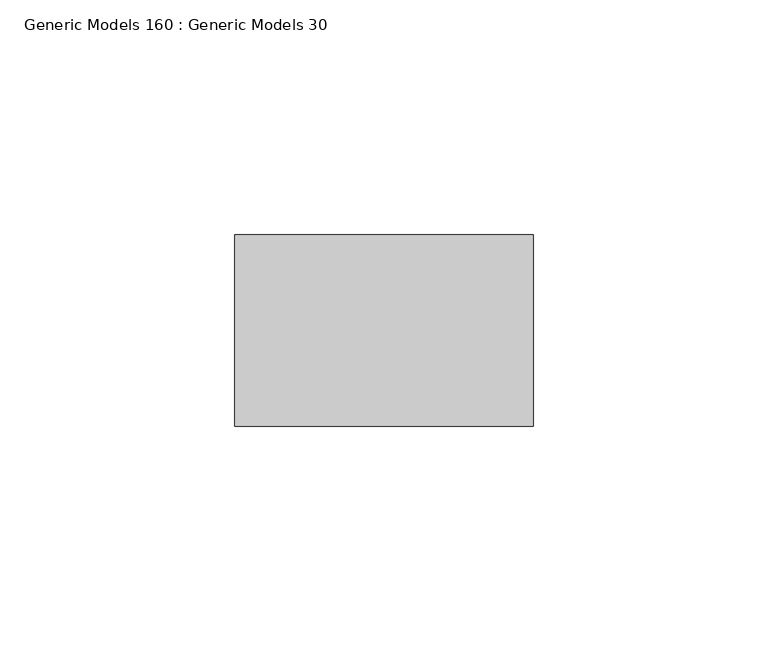
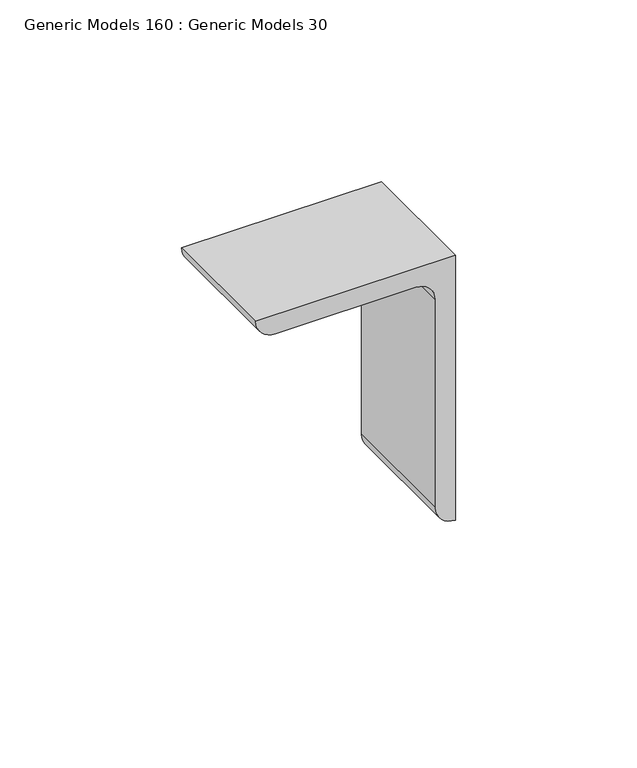
"""IFC4 building model written with IfcOpenShell, lengths in millimetres: proxy geometry, Generic Models 160 : Generic Models 30."""

from ifc_helpers import new_model, si_unit, point, frame, frame_2d, origin, place, context, project, spatial, polyline, circle_curve, trimmed, segment, composite_curve, outline, extrude, source, transform, mapped, element, save


def generic_models_160_generic_models_30_e29d707e(model_context):
    return source(origin(), model_context, "Body", "SweptSolid", [
        extrude(outline(composite_curve([segment(polyline([(268865.4044757, 33370.8340778), (268865.4044757, 33307.3340778)]), True, "CONTINUOUS"), segment(trimmed(circle_curve(frame_2d((268865.4044757, 33313.6840778)), 6.35), [point((268865.4044757, 33307.3340778))], [point((268859.0544757, 33313.6840778))], False, "CARTESIAN"), True, "CONTINUOUS"), segment(polyline([(268859.0544757, 33313.6840778), (268859.0544757, 33358.1340778)]), True, "CONTINUOUS"), segment(trimmed(circle_curve(frame_2d((268852.7044757, 33358.1340778)), 6.35), [point((268859.0544757, 33358.1340778))], [point((268852.7044757, 33364.4840778))], True, "CARTESIAN"), True, "CONTINUOUS"), segment(polyline([(268852.7044757, 33364.4840778), (268782.8544757, 33364.4840778)]), True, "CONTINUOUS"), segment(trimmed(circle_curve(frame_2d((268782.8544757, 33370.8340778)), 6.35), [point((268782.8544757, 33364.4840778))], [point((268776.5044757, 33370.8340778))], False, "CARTESIAN"), True, "CONTINUOUS"), segment(polyline([(268776.5044757, 33370.8340778), (268865.4044757, 33370.8340778)]), True, "CONTINUOUS")], self_intersect=False)), frame((0.0, 41007.6196612, 0.0), z_axis=(0.0, 1.0, 0.0), x_axis=(0.0, 0.0, 1.0)), (0.0, 0.0, 1.0), 40.7035),
    ])


if __name__ == "__main__":
    model = new_model("IFC4")
    model_context = context("Model", 3, world=origin())
    ifc_project = project(units=[si_unit("LENGTHUNIT", "METRE", prefix="MILLI")], contexts=[model_context])
    site = spatial("IfcSite", under=ifc_project)
    building = spatial("IfcBuilding", under=site)
    placement = place(None, origin())
    generic_models_160_generic_models_30_shape = generic_models_160_generic_models_30_e29d707e(model_context)
    element("IfcBuildingElementProxy", 1, Name="Generic Models 160 : Generic Models 30", ObjectType="Generic Models 160 : Generic Models 30", at=placement, inside=building, context=model_context, shape_type="MappedRepresentation", body=[
        mapped(generic_models_160_generic_models_30_shape, transform((0.0, 0.0, 0.0), x_axis=(1.0, 0.0, 0.0), y_axis=(0.0, 1.0, 0.0), z_axis=(0.0, 0.0, 1.0))),
    ])
    save(model, "model.ifc")

# Revit data of these elements
# Element 1 (IfcBuildingElementProxy, "Generic Models 160 : Generic Models 30")
#   Materials on its faces: "GALV 3 1/2\"X 2 1/2\" X 1/4\" STEEL ANGLE - WELD TO VERTICAL STEEL ANGLE"
# Materials
#   "GALV 3 1/2\"X 2 1/2\" X 1/4\" STEEL ANGLE - WELD TO VERTICAL STEEL ANGLE": class "Metal", colour RGB 199 199 199, transparency 0, Description = "Structural steel, ASTM A36 Grade B, mill finish", Cost = 0
